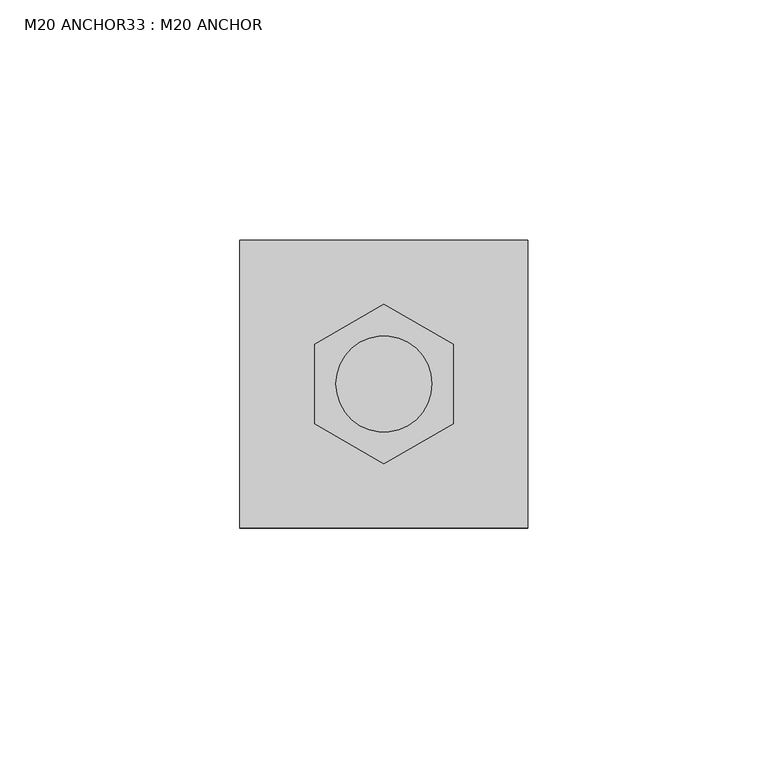
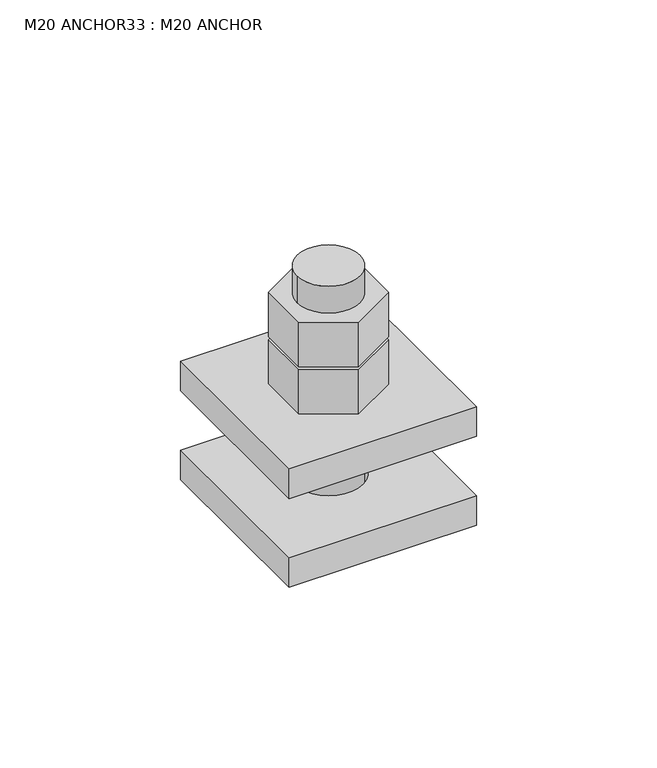
"""IFC4 building model written with IfcOpenShell, lengths in millimetres: fastener geometry, M20 ANCHOR33 : M20 ANCHOR."""

from ifc_helpers import new_model, si_unit, point, frame, frame_2d, origin, place, context, project, spatial, polyline, circle_curve, trimmed, segment, composite_curve, outline, extrude, source, transform, mapped, element, save


def m20_anchor33_m20_anchor_82ed35be(model_context):
    return source(origin(), model_context, "Body", "SweptSolid", [
        extrude(outline(polyline([(-8.0855968, 25545.0952779), (-8.0855968, 25528.4582151), (-22.4937158, 25520.1396837), (-36.9018348, 25528.4582151), (-36.9018348, 25545.0952779), (-22.4937158, 25553.4138093), (-8.0855968, 25545.0952779)]), holes=[composite_curve([segment(trimmed(circle_curve(frame_2d((-22.4937158, 25536.7767465)), 10.0), [point((-32.4937158, 25536.7767465))], [point((-12.4937158, 25536.7767465))], True, "CARTESIAN"), True, "CONTINUOUS"), segment(trimmed(circle_curve(frame_2d((-22.4937158, 25536.7767465)), 10.0), [point((-12.4937158, 25536.7767465))], [point((-32.4937158, 25536.7767465))], True, "CARTESIAN"), True, "CONTINUOUS")], self_intersect=False)]), frame((0.0, 0.0, 246.0), z_axis=(0.0, 0.0, 1.0), x_axis=(1.0, 0.0, 0.0)), (0.0, 0.0, 1.0), 15.0),
        extrude(outline(polyline([(-8.0855968, 25545.0952779), (-8.0855968, 25528.4582151), (-22.4937158, 25520.1396837), (-36.9018348, 25528.4582151), (-36.9018348, 25545.0952779), (-22.4937158, 25553.4138093), (-8.0855968, 25545.0952779)]), holes=[composite_curve([segment(trimmed(circle_curve(frame_2d((-22.4937158, 25536.7767465)), 10.0), [point((-32.4937158, 25536.7767465))], [point((-12.4937158, 25536.7767465))], True, "CARTESIAN"), True, "CONTINUOUS"), segment(trimmed(circle_curve(frame_2d((-22.4937158, 25536.7767465)), 10.0), [point((-12.4937158, 25536.7767465))], [point((-32.4937158, 25536.7767465))], True, "CARTESIAN"), True, "CONTINUOUS")], self_intersect=False)]), frame((0.0, 0.0, 230.0), z_axis=(0.0, 0.0, 1.0), x_axis=(1.0, 0.0, 0.0)), (0.0, 0.0, 1.0), 15.0),
        extrude(outline(composite_curve([segment(trimmed(circle_curve(frame_2d((-22.4937158, 25536.7767465)), 10.0), [point((-32.4937158, 25536.7767465))], [point((-12.4937158, 25536.7767465))], False, "CARTESIAN"), True, "CONTINUOUS"), segment(trimmed(circle_curve(frame_2d((-22.4937158, 25536.7767465)), 10.0), [point((-12.4937158, 25536.7767465))], [point((-32.4937158, 25536.7767465))], False, "CARTESIAN"), True, "CONTINUOUS")], self_intersect=False)), frame((0.0, 0.0, 190.0), z_axis=(0.0, 0.0, 1.0), x_axis=(1.0, 0.0, 0.0)), (0.0, 0.0, 1.0), 80.0),
        extrude(outline(polyline([(7.5062842, 25566.7767465), (7.5062842, 25506.7767465), (-52.4937158, 25506.7767465), (-52.4937158, 25566.7767465), (7.5062842, 25566.7767465)]), holes=[composite_curve([segment(trimmed(circle_curve(frame_2d((-22.4937158, 25536.7767465)), 11.0), [point((-33.4937158, 25536.7767465))], [point((-11.4937158, 25536.7767465))], True, "CARTESIAN"), True, "CONTINUOUS"), segment(trimmed(circle_curve(frame_2d((-22.4937158, 25536.7767465)), 11.0), [point((-11.4937158, 25536.7767465))], [point((-33.4937158, 25536.7767465))], True, "CARTESIAN"), True, "CONTINUOUS")], self_intersect=False)]), frame((0.0, 0.0, 190.0), z_axis=(0.0, 0.0, 1.0), x_axis=(1.0, 0.0, 0.0)), (0.0, 0.0, 1.0), 10.0),
        extrude(outline(polyline([(7.5062842, 25566.7767465), (7.5062842, 25506.7767465), (-52.4937158, 25506.7767465), (-52.4937158, 25566.7767465), (7.5062842, 25566.7767465)]), holes=[composite_curve([segment(trimmed(circle_curve(frame_2d((-22.4937158, 25536.7767465)), 11.0), [point((-33.4937158, 25536.7767465))], [point((-11.4937158, 25536.7767465))], True, "CARTESIAN"), True, "CONTINUOUS"), segment(trimmed(circle_curve(frame_2d((-22.4937158, 25536.7767465)), 11.0), [point((-11.4937158, 25536.7767465))], [point((-33.4937158, 25536.7767465))], True, "CARTESIAN"), True, "CONTINUOUS")], self_intersect=False)]), frame((0.0, 0.0, 220.0), z_axis=(0.0, 0.0, 1.0), x_axis=(1.0, 0.0, 0.0)), (0.0, 0.0, 1.0), 10.0),
    ])


if __name__ == "__main__":
    model = new_model("IFC4")
    model_context = context("Model", 3, world=origin())
    ifc_project = project(units=[si_unit("LENGTHUNIT", "METRE", prefix="MILLI")], contexts=[model_context])
    site = spatial("IfcSite", under=ifc_project)
    building = spatial("IfcBuilding", under=site)
    placement = place(None, origin())
    m20_anchor33_m20_anchor_shape = m20_anchor33_m20_anchor_82ed35be(model_context)
    element("IfcFastener", 1, ObjectType="M20 ANCHOR33 : M20 ANCHOR", at=placement, inside=building, context=model_context, shape_type="MappedRepresentation", body=[
        mapped(m20_anchor33_m20_anchor_shape, transform((0.0, 0.0, 0.0), x_axis=(1.0, 0.0, 0.0), y_axis=(0.0, 1.0, 0.0), z_axis=(0.0, 0.0, 1.0))),
    ])
    save(model, "model.ifc")
